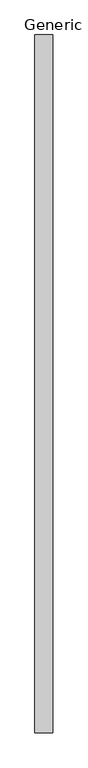
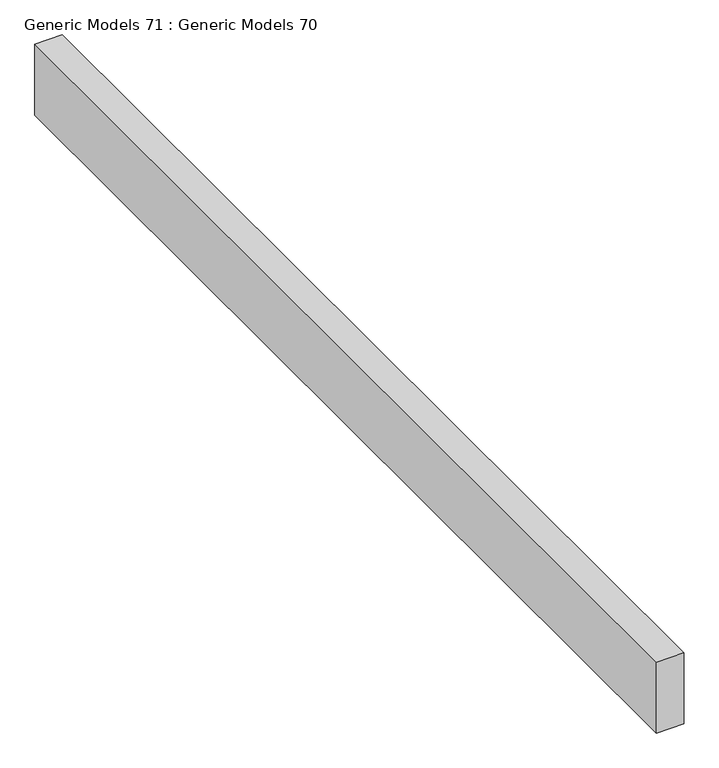
"""IFC4 building model written with IfcOpenShell, lengths in millimetres: proxy geometry, Generic Models 71 : Generic Models 70."""

from ifc_helpers import new_model, si_unit, frame, origin, place, context, project, spatial, polyline, outline, extrude, source, transform, mapped, element, save


def generic_models_71_generic_models_70_2c242a35(model_context):
    return source(origin(), model_context, "Body", "SweptSolid", [
        extrude(outline(polyline([(32192.9090778, 36321.6957942), (32192.9090778, 30860.0656612), (32053.2090778, 30860.0656612), (32053.2090778, 36321.6957942), (32192.9090778, 36321.6957942)])), frame((0.0, 0.0, 268757.4), z_axis=(0.0, 0.0, 1.0), x_axis=(1.0, 0.0, 0.0)), (0.0, 0.0, 1.0), 381.0),
    ])


if __name__ == "__main__":
    model = new_model("IFC4")
    model_context = context("Model", 3, world=origin())
    ifc_project = project(units=[si_unit("LENGTHUNIT", "METRE", prefix="MILLI")], contexts=[model_context])
    site = spatial("IfcSite", under=ifc_project)
    building = spatial("IfcBuilding", under=site)
    placement = place(None, origin())
    generic_models_71_generic_models_70_shape = generic_models_71_generic_models_70_2c242a35(model_context)
    element("IfcBuildingElementProxy", 1, Name="Generic Models 71 : Generic Models 70", ObjectType="Generic Models 71 : Generic Models 70", at=placement, inside=building, context=model_context, shape_type="MappedRepresentation", body=[
        mapped(generic_models_71_generic_models_70_shape, transform((0.0, 0.0, 0.0), x_axis=(1.0, 0.0, 0.0), y_axis=(0.0, 1.0, 0.0), z_axis=(0.0, 0.0, 1.0))),
    ])
    save(model, "model.ifc")

# Revit data of these elements
# Element 1 (IfcBuildingElementProxy, "Generic Models 71 : Generic Models 70")
#   Materials on its faces: "5 1/2\" x 15\" GLULAM BEAM"
# Materials
#   "5 1/2\" x 15\" GLULAM BEAM": class "Wood", colour RGB 112 64 44, transparency 0, Description = "Pinus Echinata", Cost = 0
